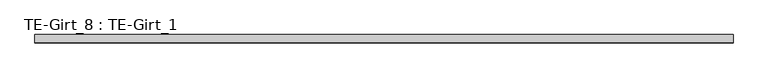
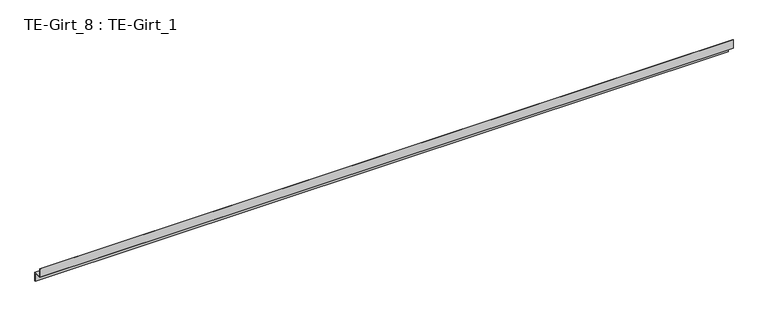
"""IFC4 building model written with IfcOpenShell, lengths in millimetres: proxy geometry, TE-Girt_8 : TE-Girt_1."""

from ifc_helpers import new_model, si_unit, frame, origin, place, context, project, spatial, polyline, outline, extrude, source, transform, mapped, element, save


def te_girt_8_te_girt_1_d8d35839(model_context):
    return source(origin(), model_context, "Body", "SweptSolid", [
        extrude(outline(polyline([(-531639.2163841, 1657.35), (-531639.2163841, 1619.25), (-531640.1093528, 1619.25), (-531640.1093528, 1656.4570312), (-531674.1249348, 1656.4570312), (-531674.1249348, 1694.5570312), (-531673.231966, 1694.5570312), (-531673.231966, 1657.35), (-531639.2163841, 1657.35)])), frame((587397.6434739, 0.0, 0.0), z_axis=(1.0, 0.0, 0.0), x_axis=(0.0, 1.0, 0.0)), (0.0, 0.0, 1.0), 2921.0),
    ])


if __name__ == "__main__":
    model = new_model("IFC4")
    model_context = context("Model", 3, world=origin())
    ifc_project = project(units=[si_unit("LENGTHUNIT", "METRE", prefix="MILLI")], contexts=[model_context])
    site = spatial("IfcSite", under=ifc_project)
    building = spatial("IfcBuilding", under=site)
    placement = place(None, origin())
    te_girt_8_te_girt_1_shape = te_girt_8_te_girt_1_d8d35839(model_context)
    element("IfcBuildingElementProxy", 1, Name="TE-Girt_8 : TE-Girt_1", ObjectType="TE-Girt_8 : TE-Girt_1", at=placement, inside=building, context=model_context, shape_type="MappedRepresentation", body=[
        mapped(te_girt_8_te_girt_1_shape, transform((0.0, 0.0, 0.0), x_axis=(1.0, 0.0, 0.0), y_axis=(0.0, 1.0, 0.0), z_axis=(0.0, 0.0, 1.0))),
    ])
    save(model, "model.ifc")

# Revit data of these elements
# Element 1 (IfcBuildingElementProxy, "TE-Girt_8 : TE-Girt_1")
#   Materials on its faces: "Z-FURRING, COLD-FORMED GALV."
# Materials
#   "Z-FURRING, COLD-FORMED GALV.": class "Generic", colour RGB 143 142 141, transparency 0, Cost = 0
